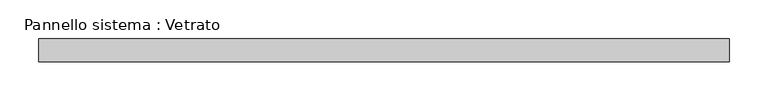
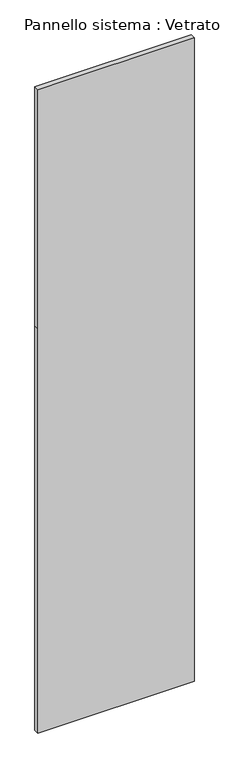
"""IFC4 building model written with IfcOpenShell, lengths in millimetres: plate geometry, Pannello sistema : Vetrato."""

from ifc_helpers import new_model, si_unit, frame, origin, place, context, project, spatial, polyline, outline, extrude, source, transform, mapped, element, save


def pannello_sistema_vetrato_00c806ab(model_context):
    return source(origin(), model_context, "Body", "SweptSolid", [
        extrude(outline(polyline([(0.0, -447.5), (0.0, 447.5), (2450.0, 447.5), (3900.0, 447.5), (3900.0, -447.5), (2450.0, -447.5), (0.0, -447.5)])), frame((0.0, -15.0, 0.0), z_axis=(0.0, 1.0, 0.0), x_axis=(0.0, 0.0, 1.0)), (0.0, 0.0, 1.0), 30.0),
    ])


if __name__ == "__main__":
    model = new_model("IFC4")
    model_context = context("Model", 3, world=origin())
    ifc_project = project(units=[si_unit("LENGTHUNIT", "METRE", prefix="MILLI")], contexts=[model_context])
    site = spatial("IfcSite", under=ifc_project)
    building = spatial("IfcBuilding", under=site)
    placement = place(None, origin())
    pannello_sistema_vetrato_shape = pannello_sistema_vetrato_00c806ab(model_context)
    element("IfcPlate", 1, ObjectType="Pannello sistema : Vetrato", at=placement, inside=building, context=model_context, shape_type="MappedRepresentation", body=[
        mapped(pannello_sistema_vetrato_shape, transform((0.0, 0.0, 0.0), x_axis=(1.0, 0.0, 0.0), y_axis=(0.0, 1.0, 0.0), z_axis=(0.0, 0.0, 1.0))),
    ])
    save(model, "model.ifc")

# Revit data of these elements
# Type "Pannello sistema : Vetrato"
#   Construction Type Id = "GSP4R"
#   Analytic Construction = "Vetrata singola Pilkington 1/8 in"
#   Visual Light Transmittance = 0.9
#   Solar Heat Gain Coefficient = 0.86
#   Heat Transfer Coefficient (U) = 6.7069 W/(m²·K)
# Element 1 (IfcPlate, "Pannello sistema : Vetrato")
#   Materials on its faces: "Default - Vetro"
# Materials
#   "Default - Vetro": class "Vetro", colour RGB 208 208 208, transparency 0.7, Cost = 0
